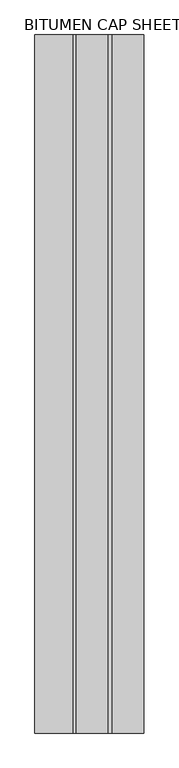
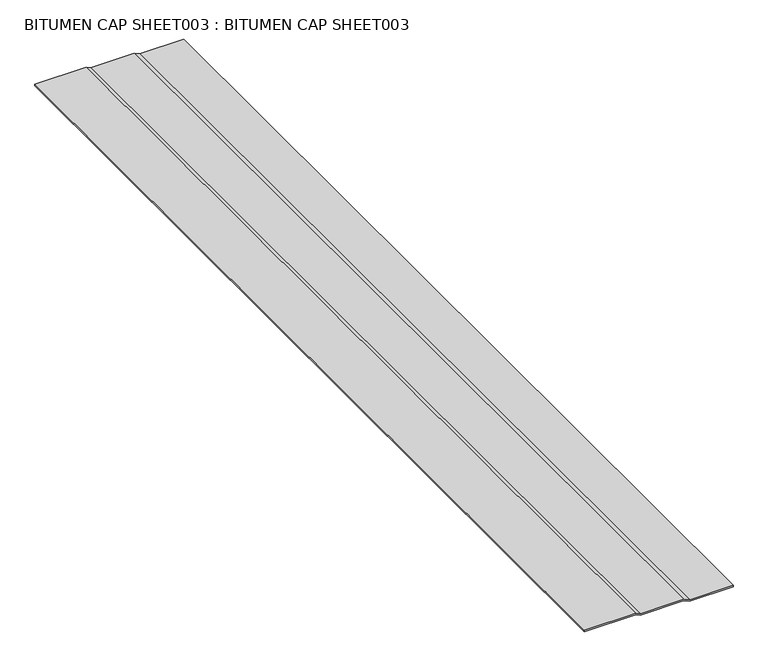
"""IFC4 building model written with IfcOpenShell, lengths in millimetres: proxy geometry, BITUMEN CAP SHEET003 : BITUMEN CAP SHEET003."""

from ifc_helpers import new_model, si_unit, frame, origin, place, context, project, spatial, polyline, outline, extrude, source, transform, mapped, element, save


def bitumen_cap_sheet003_bitumen_cap_sheet003_03d49bda(model_context):
    return source(origin(), model_context, "Body", "SweptSolid", [
        extrude(outline(polyline([(40259.2002678, -2469.2761954), (40262.3752678, -2469.2761954), (40262.3752678, -2560.795457), (40267.6612773, -2573.2602756), (40267.6612773, -2663.9440313), (40271.9940719, -2673.6609328), (40271.9940719, -2781.5474293), (40268.8188423, -2781.5474293), (40268.8188423, -2674.3362183), (40264.4862773, -2664.6198318), (40264.4862773, -2573.9056756), (40259.2002678, -2561.440857), (40259.2002678, -2469.2761954)])), frame((0.0, 999.75, 0.0), z_axis=(0.0, 1.0, 0.0), x_axis=(0.0, 0.0, 1.0)), (0.0, 0.0, 1.0), 2000.25),
    ])


if __name__ == "__main__":
    model = new_model("IFC4")
    model_context = context("Model", 3, world=origin())
    ifc_project = project(units=[si_unit("LENGTHUNIT", "METRE", prefix="MILLI")], contexts=[model_context])
    site = spatial("IfcSite", under=ifc_project)
    building = spatial("IfcBuilding", under=site)
    placement = place(None, origin())
    bitumen_cap_sheet003_bitumen_cap_sheet003_shape = bitumen_cap_sheet003_bitumen_cap_sheet003_03d49bda(model_context)
    element("IfcBuildingElementProxy", 1, Name="BITUMEN CAP SHEET003 : BITUMEN CAP SHEET003", ObjectType="BITUMEN CAP SHEET003 : BITUMEN CAP SHEET003", at=placement, inside=building, context=model_context, shape_type="MappedRepresentation", body=[
        mapped(bitumen_cap_sheet003_bitumen_cap_sheet003_shape, transform((0.0, 0.0, 0.0), x_axis=(1.0, 0.0, 0.0), y_axis=(0.0, 1.0, 0.0), z_axis=(0.0, 0.0, 1.0))),
    ])
    save(model, "model.ifc")

# Revit data of these elements
# Type "BITUMEN CAP SHEET003 : BITUMEN CAP SHEET003"
#   NameOverride = "BITUMEN CAP SHEET003"
# Element 1 (IfcBuildingElementProxy, "BITUMEN CAP SHEET003 : BITUMEN CAP SHEET003")
#   Materials on its faces: "MODIFIED BITUMEN GRANULE SURFACED CAP SHEET"
# Materials
#   "MODIFIED BITUMEN GRANULE SURFACED CAP SHEET": class "Unassigned", colour RGB 85 85 127, transparency 0
